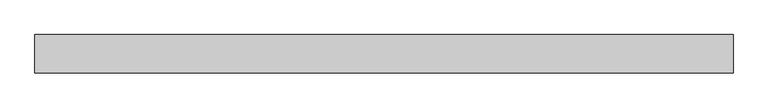
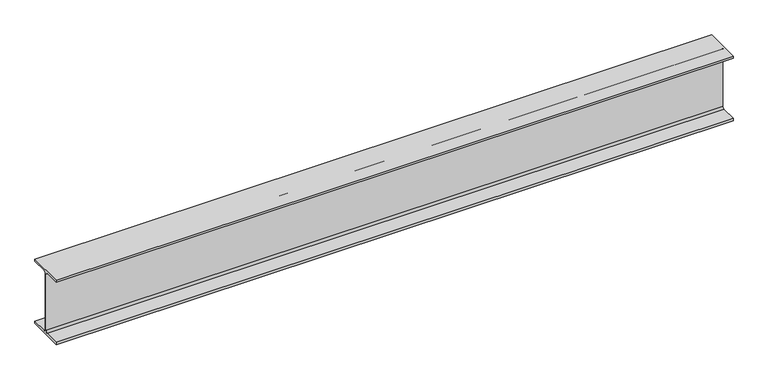
"""IFC4 building model written with IfcOpenShell, lengths in millimetres: beam geometry, Old_Steel Beam_H-KSD3502 : H_SB_ASB_H-200×200x8x12."""

from ifc_helpers import new_model, si_unit, point, frame, frame_2d, origin, place, context, project, spatial, polyline, circle_curve, trimmed, segment, composite_curve, outline, extrude, source, transform, mapped, element, save


def beam_69cf824f(model_context):
    return source(origin(), model_context, "Body", "SweptSolid", [
        extrude(outline(composite_curve([segment(polyline([(82.5, -141.5), (82.5, -151.7), (-82.5, -151.7), (-82.5, -141.5), (-11.9, -141.5)]), True, "CONTINUOUS"), segment(trimmed(circle_curve(frame_2d((-11.9, -132.6)), 8.9), [point((-11.9, -141.5))], [point((-3.0, -132.6))], True, "CARTESIAN"), True, "CONTINUOUS"), segment(polyline([(-3.0, -132.6), (-3.0, 132.6)]), True, "CONTINUOUS"), segment(trimmed(circle_curve(frame_2d((-11.9, 132.6)), 8.9), [point((-3.0, 132.6))], [point((-11.9, 141.5))], True, "CARTESIAN"), True, "CONTINUOUS"), segment(polyline([(-11.9, 141.5), (-82.5, 141.5), (-82.5, 151.7), (82.5, 151.7), (82.5, 141.5), (11.9, 141.5)]), True, "CONTINUOUS"), segment(trimmed(circle_curve(frame_2d((11.9, 132.6)), 8.9), [point((11.9, 141.5))], [point((3.0, 132.6))], True, "CARTESIAN"), True, "CONTINUOUS"), segment(polyline([(3.0, 132.6), (3.0, -132.6)]), True, "CONTINUOUS"), segment(trimmed(circle_curve(frame_2d((11.9, -132.6)), 8.9), [point((3.0, -132.6))], [point((11.9, -141.5))], True, "CARTESIAN"), True, "CONTINUOUS"), segment(polyline([(11.9, -141.5), (82.5, -141.5)]), True, "CONTINUOUS")], self_intersect=False)), frame((-1318.7999205, 0.0, 0.0), z_axis=(1.0, 0.0, 0.0), x_axis=(0.0, 1.0, 0.0)), (0.0, 0.0, 1.0), 3016.4229709),
    ])


if __name__ == "__main__":
    model = new_model("IFC4")
    model_context = context("Model", 3, world=origin())
    ifc_project = project(units=[si_unit("LENGTHUNIT", "METRE", prefix="MILLI")], contexts=[model_context])
    site = spatial("IfcSite", under=ifc_project)
    building = spatial("IfcBuilding", under=site)
    placement = place(None, origin())
    beam_shape = beam_69cf824f(model_context)
    element("IfcBeam", 1, ObjectType="Old_Steel Beam_H-KSD3502 : H_SB_ASB_H-200×200x8x12", at=placement, inside=building, context=model_context, shape_type="MappedRepresentation", body=[
        mapped(beam_shape, transform((0.0, 0.0, 0.0), x_axis=(1.0, 0.0, 0.0), y_axis=(0.0, 1.0, 0.0), z_axis=(0.0, 0.0, 1.0))),
    ])
    save(model, "model.ifc")

# Revit data of these elements
# Type "Old_Steel Beam_H-KSD3502 : H_SB_ASB_H-200×200x8x12"
#   Width = 20.0 cm
#   Web Thickness = 0.8 cm
#   Web Fillet = 1.3 cm
#   Warping Constant = 141376.0 cm⁶
#   Torsional Moment of Inertia = 26.2485 cm⁴
#   Torsional Modulus = 1.0 cm³
#   Section Area = 63.53 cm²
#   Plastic Modulus weak axis = 244.0 cm³
#   Plastic Modulus strong axis = 525.0 cm³
#   Perimeter = 1.16 m²/m
#   Nominal Weight = 49.90 kgf/m
#   Moment of Inertia weak axis = 1600.00 cm⁴
#   Moment of Inertia strong axis = 4720.00 cm⁴
#   Height = 20.0 cm
#   Flange Thickness = 1.2 cm
#   Elastic Modulus weak axis = 160.0 cm³
#   Elastic Modulus strong axis = 472.0 cm³
#   Centroid Vertical = 10.0 cm
#   Centroid Horizontal = 10.0 cm
#   Length [instance default] = 1.5240 m
#   Structural Material [instance default] = Steel, 45-345
#   Assembly Code = ""
# Element 1 (IfcBeam, "Old_Steel Beam_H-KSD3502 : H_SB_ASB_H-200×200x8x12")
#   Structural Material = none
# Materials
#   "Steel, 45-345": class "Metal", colour RGB 189 187 185, transparency 0, Description = "Steel 345 MPa", Cost = 0
